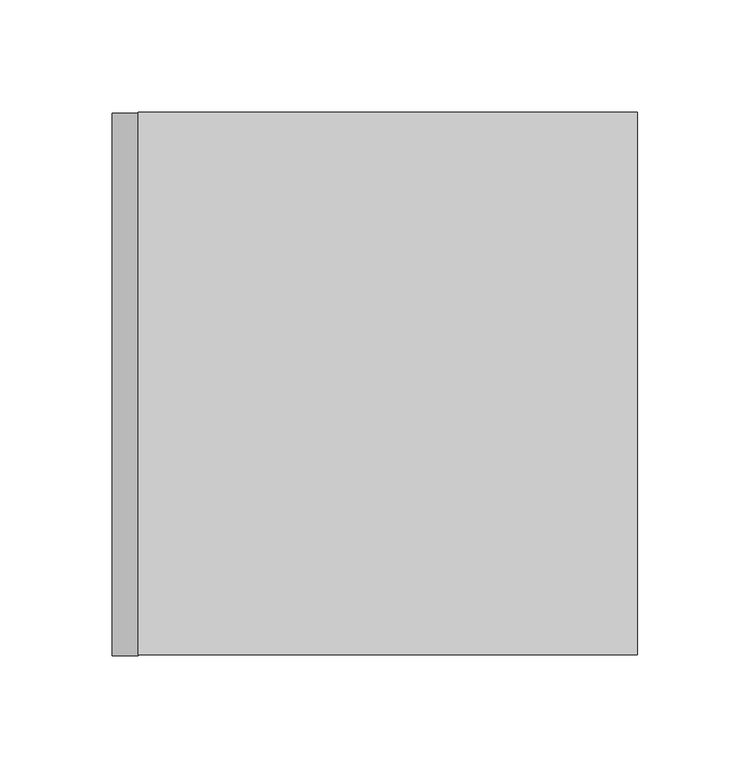
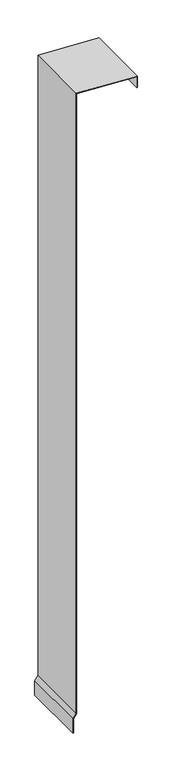
"""IFC4 building model written with IfcOpenShell, lengths in millimetres: proxy geometry, Generic Models 7:Generic Models 1:5:Generic Models 1:5 : Generic Models 7:Generic Models 1:337419:11 : Generic Models 7:Generic Models 1:5:Generic Models 1:5 : Generic Models 7:Generic Models 1:337419:311462."""

import ifcopenshell
import ifcopenshell.guid

model = None  # the IFC model being written
_history = None  # IfcOwnerHistory: only IFC2X3 demands one
_inside = {}  # id of a spatial element -> (the spatial element, [elements in it])
_under = {}  # id of a project, library or spatial element -> (it, [spatial elements below it])
_declared = {}  # id of a project -> (the project, [libraries it declares])
_typed = {}  # id of a type object -> (the type object, [elements of that type])
_made_of = {}  # id of a material, layer set ... -> (it, [elements and type objects made of it])


def new_model(schema):
    """Start an empty IFC model of exactly this schema.

    Asked for "IFC4X3", IfcOpenShell would pick the latest addendum, in which some entities
    have other attributes; the version numbers below select the first issue.
    IFC2X3 requires an IfcOwnerHistory on every rooted entity: one is made here for all.
    """
    global model, _history
    if schema == "IFC4X3":
        model = ifcopenshell.file(schema_version=(4, 3, 0, 0))
    else:
        model = ifcopenshell.file(schema=schema)
    _inside.clear()
    _under.clear()
    _declared.clear()
    _typed.clear()
    _made_of.clear()
    _history = None
    if model.schema == "IFC2X3":
        org = make("IfcOrganization", Name="unknown")
        user = make(
            "IfcPersonAndOrganization",
            ThePerson=make("IfcPerson", FamilyName="unknown"),
            TheOrganization=org,
        )
        app = make(
            "IfcApplication",
            ApplicationDeveloper=org,
            Version="unknown",
            ApplicationFullName="unknown",
            ApplicationIdentifier="unknown",
        )
        _history = make(
            "IfcOwnerHistory",
            OwningUser=user,
            OwningApplication=app,
            ChangeAction="ADDED",
            CreationDate=0,
        )
    return model


def make(cls, **values):
    """One entity of the class cls with the attributes given. An attribute that is None is left unset."""
    return model.create_entity(
        cls, **{name: value for name, value in values.items() if value is not None}
    )


def rooted(cls, **values):
    """An entity with a GlobalId (a new one), such as an element, a storey or a relation."""
    return make(cls, GlobalId=ifcopenshell.guid.new(), OwnerHistory=_history, **values)


def si_unit(unit_type, name, prefix=None):
    """IfcSIUnit, for example si_unit("LENGTHUNIT", "METRE", prefix="MILLI")."""
    return make("IfcSIUnit", UnitType=unit_type, Prefix=prefix, Name=name)


def assignment(units):
    """IfcUnitAssignment: the units of a project."""
    return None if units is None else make("IfcUnitAssignment", Units=units)


def point(xyz):
    """IfcCartesianPoint."""
    return None if xyz is None else make("IfcCartesianPoint", Coordinates=xyz)


def direction(xyz):
    """IfcDirection."""
    return None if xyz is None else make("IfcDirection", DirectionRatios=xyz)


def frame(location, z_axis=None, x_axis=None):
    """IfcAxis2Placement3D, a coordinate frame: its origin and axes. An axis left out is left unset."""
    return make(
        "IfcAxis2Placement3D",
        Location=point(location),
        Axis=direction(z_axis),
        RefDirection=direction(x_axis),
    )


def origin():
    """The frame at (0, 0, 0) with its axes left unset."""
    return frame((0.0, 0.0, 0.0))


def place(relative_to, where):
    """IfcLocalPlacement: puts the frame where relative to a parent placement (None: the world)."""
    return make(
        "IfcLocalPlacement", PlacementRelTo=relative_to, RelativePlacement=where
    )


def context(
    kind, dimensions, precision=None, world=None, true_north=None, identifier=None
):
    """IfcGeometricRepresentationContext, for example the 3D "Model" context."""
    return make(
        "IfcGeometricRepresentationContext",
        ContextIdentifier=identifier,
        ContextType=kind,
        CoordinateSpaceDimension=dimensions,
        Precision=precision,
        WorldCoordinateSystem=world,
        TrueNorth=true_north,
    )


def project(units=None, contexts=None):
    """IfcProject with its units and contexts."""
    return rooted(
        "IfcProject",
        Name="project",
        RepresentationContexts=contexts,
        UnitsInContext=assignment(units),
    )


def spatial(cls, under=None, at=None, **own):
    """A site, building, storey or space (cls), placed at a placement, below another one or the project."""
    s = rooted(cls, ObjectPlacement=at, **own)
    if under is not None:
        _under.setdefault(under.id(), (under, []))[1].append(s)
    return s


def polyline(points):
    """IfcPolyline through the points."""
    return make("IfcPolyline", Points=[point(p) for p in points])


def outline(outer, holes=None, kind="AREA"):
    """IfcArbitraryClosedProfileDef: a profile drawn as a closed curve; with holes, ...WithVoids."""
    if holes is None:
        return make("IfcArbitraryClosedProfileDef", ProfileType=kind, OuterCurve=outer)
    return make(
        "IfcArbitraryProfileDefWithVoids",
        ProfileType=kind,
        OuterCurve=outer,
        InnerCurves=holes,
    )


def extrude(swept, where, along, depth):
    """IfcExtrudedAreaSolid: the profile swept, set in the frame where, extruded along a direction by depth."""
    return make(
        "IfcExtrudedAreaSolid",
        SweptArea=swept,
        Position=where,
        ExtrudedDirection=direction(along),
        Depth=depth,
    )


def shape(context_of_items, identifier, shape_type, items):
    """IfcShapeRepresentation: the items that make up one representation, for example the "Body"."""
    return make(
        "IfcShapeRepresentation",
        ContextOfItems=context_of_items,
        RepresentationIdentifier=identifier,
        RepresentationType=shape_type,
        Items=items,
    )


def source(mapping_origin, context_of_items, identifier, shape_type, items):
    """IfcRepresentationMap: a shape defined once, which mapped items show again and again."""
    return make(
        "IfcRepresentationMap",
        MappingOrigin=mapping_origin,
        MappedRepresentation=shape(context_of_items, identifier, shape_type, items),
    )


def transform(
    local_origin,
    x_axis=None,
    y_axis=None,
    z_axis=None,
    scale=None,
    scale2=None,
    scale3=None,
    uniform=True,
):
    """IfcCartesianTransformationOperator3D, or its non-uniform kind. x_axis, y_axis, z_axis: its Axis1, 2, 3."""
    if uniform:
        return make(
            "IfcCartesianTransformationOperator3D",
            Axis1=direction(x_axis),
            Axis2=direction(y_axis),
            LocalOrigin=point(local_origin),
            Scale=scale,
            Axis3=direction(z_axis),
        )
    return make(
        "IfcCartesianTransformationOperator3DnonUniform",
        Axis1=direction(x_axis),
        Axis2=direction(y_axis),
        LocalOrigin=point(local_origin),
        Scale=scale,
        Axis3=direction(z_axis),
        Scale2=scale2,
        Scale3=scale3,
    )


def mapped(mapping_source, mapping_target):
    """IfcMappedItem: shows the shape of a source again, moved by a transform."""
    return make(
        "IfcMappedItem", MappingSource=mapping_source, MappingTarget=mapping_target
    )


def made_of(thing, what):
    """Note that an element or type object is made of a material, layer set ...; save() writes the relation."""
    if what is not None:
        _made_of.setdefault(what.id(), (what, []))[1].append(thing)
    return thing


def element(
    cls,
    number,
    at=None,
    inside=None,
    cuts=None,
    type_object=None,
    material=None,
    context=None,
    identifier="Body",
    shape_type=None,
    held_by="IfcProductDefinitionShape",
    body=None,
    shapes=None,
    **own,
):
    """One element of the class cls, such as IfcWall. Its Tag is "e" and its number.

    at: its placement. inside: the storey or other place that contains it. cuts: it is an
    opening in that element (IfcRelVoidsElement). A single representation is given by context,
    identifier, shape_type and body (its items); several are given by shapes. held_by: the class
    of the entity that holds the representations. save() writes the other relations.
    """
    e = rooted(cls, Tag="e%d" % number, ObjectPlacement=at, **own)
    if body is not None:
        shapes = [shape(context, identifier, shape_type, body)]
    if shapes is not None:
        e.Representation = make(held_by, Representations=shapes)
    if inside is not None:
        _inside.setdefault(inside.id(), (inside, []))[1].append(e)
    if cuts is not None:
        rooted(
            "IfcRelVoidsElement", RelatingBuildingElement=cuts, RelatedOpeningElement=e
        )
    if type_object is not None:
        _typed.setdefault(type_object.id(), (type_object, []))[1].append(e)
    return made_of(e, material)


def aggregate(whole, parts):
    """IfcRelAggregates: a whole, such as a stair, and the parts it consists of."""
    return rooted("IfcRelAggregates", RelatingObject=whole, RelatedObjects=parts)


def save(model, path):
    """Write the relations noted so far, then the file.

    IfcRelAggregates (storeys below a building ...), IfcRelContainedInSpatialStructure (elements
    in a storey), IfcRelDefinesByType, IfcRelAssociatesMaterial and IfcRelDeclares: one each for
    every whole, place, type object, material and project.
    """
    for whole, parts in _under.values():
        aggregate(whole, parts)
    for where, things in _inside.values():
        rooted(
            "IfcRelContainedInSpatialStructure",
            RelatedElements=things,
            RelatingStructure=where,
        )
    for kind, things in _typed.values():
        rooted("IfcRelDefinesByType", RelatedObjects=things, RelatingType=kind)
    for what, things in _made_of.values():
        rooted("IfcRelAssociatesMaterial", RelatedObjects=things, RelatingMaterial=what)
    for by, libraries in _declared.values():
        rooted("IfcRelDeclares", RelatingContext=by, RelatedDefinitions=libraries)
    model.write(path)


def generic_models_3ad6a1f5(model_context):
    return source(origin(), model_context, "Body", "SweptSolid", [
        extrude(outline(polyline([(3795.8885169, 560352.1679739), (6178.9388113, 560352.1679739), (6167.4563403, 560571.2665711), (6125.115987, 560571.2665711), (6125.115987, 560572.8540711), (6168.9628216, 560572.8540711), (6180.6116872, 560350.5804739), (3796.3890538, 560350.5804739), (3779.8619698, 560339.0080851), (3725.3283058, 560339.0080851), (3725.3283058, 560340.5955851), (3779.361433, 560340.5955851), (3795.8885169, 560352.1679739)])), frame((0.0, -579019.7413841, 0.0), z_axis=(0.0, 1.0, 0.0), x_axis=(0.0, 0.0, 1.0)), (0.0, 0.0, 1.0), 241.3),
    ])


if __name__ == "__main__":
    model = new_model("IFC4")
    model_context = context("Model", 3, world=origin())
    ifc_project = project(units=[si_unit("LENGTHUNIT", "METRE", prefix="MILLI")], contexts=[model_context])
    site = spatial("IfcSite", under=ifc_project)
    building = spatial("IfcBuilding", under=site)
    placement = place(None, origin())
    generic_models_shape = generic_models_3ad6a1f5(model_context)
    element("IfcBuildingElementProxy", 1, Name="Generic Models 7:Generic Models 1:5:Generic Models 1:5 : Generic Models 7:Generic Models 1:337419:11 : Generic Models 7:Generic Models 1:5:Generic Models 1:5 : Generic Models 7:Generic Models 1:337419:311462", ObjectType="Generic Models 7:Generic Models 1:5:Generic Models 1:5 : Generic Models 7:Generic Models 1:337419:11 : Generic Models 7:Generic Models 1:5:Generic Models 1:5 : Generic Models 7:Generic Models 1:337419:311462", at=placement, inside=building, context=model_context, shape_type="MappedRepresentation", body=[
        mapped(generic_models_shape, transform((0.0, 0.0, 0.0), x_axis=(1.0, 0.0, 0.0), y_axis=(0.0, 1.0, 0.0), z_axis=(0.0, 0.0, 1.0))),
    ])
    save(model, "model.ifc")

# Revit data of these elements
# Type "Generic Models 7:Generic Models 1:5:Generic Models 1:5 : Generic Models 7:Generic Models 1:337419:11 : Generic Models 7:Generic Models 1:5:Generic Models 1:5 : Generic Models 7:Generic Models 1:337419:311462"
#   NameOverride = "Generic Models 7:Generic Models 1:5:Generic Models 1:5 : Generic Models 7:Generic Models 1:337419:311462"
#   ObjectTypeOverride = "Generic Models 1:5 : Generic Models 7:Generic Models 1:337419"
#   Reference = "Generic Models 1"
#   Tag = "311462"
# Element 1 (IfcBuildingElementProxy, "Generic Models 7:Generic Models 1:5:Generic Models 1:5 : Generic Models 7:Generic Models 1:337419:11 : Generic Models 7:Generic Models 1:5:Generic Models 1:5 : Generic Models 7:Generic Models 1:337419:311462")
#   Materials on its faces: "UV STABLE WATER RESISTANT VAPOR PERMEABLE AIR BARRIER"
# Materials
#   "UV STABLE WATER RESISTANT VAPOR PERMEABLE AIR BARRIER": class "Generic", colour RGB 51 162 45, transparency 0, Description = "Polyethylene film membrane", Cost = 0
